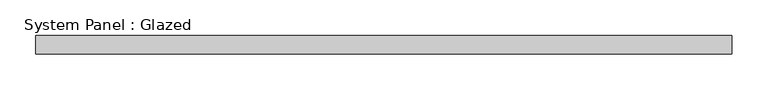
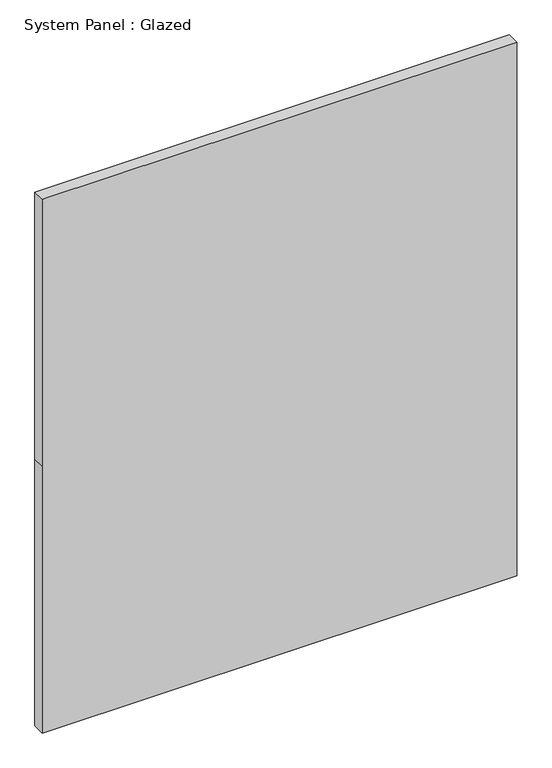
"""IFC4 building model written with IfcOpenShell, lengths in millimetres: plate geometry, System Panel : Glazed."""

import ifcopenshell
import ifcopenshell.guid

model = None  # the IFC model being written
_history = None  # IfcOwnerHistory: only IFC2X3 demands one
_inside = {}  # id of a spatial element -> (the spatial element, [elements in it])
_under = {}  # id of a project, library or spatial element -> (it, [spatial elements below it])
_declared = {}  # id of a project -> (the project, [libraries it declares])
_typed = {}  # id of a type object -> (the type object, [elements of that type])
_made_of = {}  # id of a material, layer set ... -> (it, [elements and type objects made of it])


def new_model(schema):
    """Start an empty IFC model of exactly this schema.

    Asked for "IFC4X3", IfcOpenShell would pick the latest addendum, in which some entities
    have other attributes; the version numbers below select the first issue.
    IFC2X3 requires an IfcOwnerHistory on every rooted entity: one is made here for all.
    """
    global model, _history
    if schema == "IFC4X3":
        model = ifcopenshell.file(schema_version=(4, 3, 0, 0))
    else:
        model = ifcopenshell.file(schema=schema)
    _inside.clear()
    _under.clear()
    _declared.clear()
    _typed.clear()
    _made_of.clear()
    _history = None
    if model.schema == "IFC2X3":
        org = make("IfcOrganization", Name="unknown")
        user = make(
            "IfcPersonAndOrganization",
            ThePerson=make("IfcPerson", FamilyName="unknown"),
            TheOrganization=org,
        )
        app = make(
            "IfcApplication",
            ApplicationDeveloper=org,
            Version="unknown",
            ApplicationFullName="unknown",
            ApplicationIdentifier="unknown",
        )
        _history = make(
            "IfcOwnerHistory",
            OwningUser=user,
            OwningApplication=app,
            ChangeAction="ADDED",
            CreationDate=0,
        )
    return model


def make(cls, **values):
    """One entity of the class cls with the attributes given. An attribute that is None is left unset."""
    return model.create_entity(
        cls, **{name: value for name, value in values.items() if value is not None}
    )


def rooted(cls, **values):
    """An entity with a GlobalId (a new one), such as an element, a storey or a relation."""
    return make(cls, GlobalId=ifcopenshell.guid.new(), OwnerHistory=_history, **values)


def si_unit(unit_type, name, prefix=None):
    """IfcSIUnit, for example si_unit("LENGTHUNIT", "METRE", prefix="MILLI")."""
    return make("IfcSIUnit", UnitType=unit_type, Prefix=prefix, Name=name)


def assignment(units):
    """IfcUnitAssignment: the units of a project."""
    return None if units is None else make("IfcUnitAssignment", Units=units)


def point(xyz):
    """IfcCartesianPoint."""
    return None if xyz is None else make("IfcCartesianPoint", Coordinates=xyz)


def direction(xyz):
    """IfcDirection."""
    return None if xyz is None else make("IfcDirection", DirectionRatios=xyz)


def frame(location, z_axis=None, x_axis=None):
    """IfcAxis2Placement3D, a coordinate frame: its origin and axes. An axis left out is left unset."""
    return make(
        "IfcAxis2Placement3D",
        Location=point(location),
        Axis=direction(z_axis),
        RefDirection=direction(x_axis),
    )


def origin():
    """The frame at (0, 0, 0) with its axes left unset."""
    return frame((0.0, 0.0, 0.0))


def place(relative_to, where):
    """IfcLocalPlacement: puts the frame where relative to a parent placement (None: the world)."""
    return make(
        "IfcLocalPlacement", PlacementRelTo=relative_to, RelativePlacement=where
    )


def context(
    kind, dimensions, precision=None, world=None, true_north=None, identifier=None
):
    """IfcGeometricRepresentationContext, for example the 3D "Model" context."""
    return make(
        "IfcGeometricRepresentationContext",
        ContextIdentifier=identifier,
        ContextType=kind,
        CoordinateSpaceDimension=dimensions,
        Precision=precision,
        WorldCoordinateSystem=world,
        TrueNorth=true_north,
    )


def project(units=None, contexts=None):
    """IfcProject with its units and contexts."""
    return rooted(
        "IfcProject",
        Name="project",
        RepresentationContexts=contexts,
        UnitsInContext=assignment(units),
    )


def spatial(cls, under=None, at=None, **own):
    """A site, building, storey or space (cls), placed at a placement, below another one or the project."""
    s = rooted(cls, ObjectPlacement=at, **own)
    if under is not None:
        _under.setdefault(under.id(), (under, []))[1].append(s)
    return s


def polyline(points):
    """IfcPolyline through the points."""
    return make("IfcPolyline", Points=[point(p) for p in points])


def outline(outer, holes=None, kind="AREA"):
    """IfcArbitraryClosedProfileDef: a profile drawn as a closed curve; with holes, ...WithVoids."""
    if holes is None:
        return make("IfcArbitraryClosedProfileDef", ProfileType=kind, OuterCurve=outer)
    return make(
        "IfcArbitraryProfileDefWithVoids",
        ProfileType=kind,
        OuterCurve=outer,
        InnerCurves=holes,
    )


def extrude(swept, where, along, depth):
    """IfcExtrudedAreaSolid: the profile swept, set in the frame where, extruded along a direction by depth."""
    return make(
        "IfcExtrudedAreaSolid",
        SweptArea=swept,
        Position=where,
        ExtrudedDirection=direction(along),
        Depth=depth,
    )


def shape(context_of_items, identifier, shape_type, items):
    """IfcShapeRepresentation: the items that make up one representation, for example the "Body"."""
    return make(
        "IfcShapeRepresentation",
        ContextOfItems=context_of_items,
        RepresentationIdentifier=identifier,
        RepresentationType=shape_type,
        Items=items,
    )


def source(mapping_origin, context_of_items, identifier, shape_type, items):
    """IfcRepresentationMap: a shape defined once, which mapped items show again and again."""
    return make(
        "IfcRepresentationMap",
        MappingOrigin=mapping_origin,
        MappedRepresentation=shape(context_of_items, identifier, shape_type, items),
    )


def transform(
    local_origin,
    x_axis=None,
    y_axis=None,
    z_axis=None,
    scale=None,
    scale2=None,
    scale3=None,
    uniform=True,
):
    """IfcCartesianTransformationOperator3D, or its non-uniform kind. x_axis, y_axis, z_axis: its Axis1, 2, 3."""
    if uniform:
        return make(
            "IfcCartesianTransformationOperator3D",
            Axis1=direction(x_axis),
            Axis2=direction(y_axis),
            LocalOrigin=point(local_origin),
            Scale=scale,
            Axis3=direction(z_axis),
        )
    return make(
        "IfcCartesianTransformationOperator3DnonUniform",
        Axis1=direction(x_axis),
        Axis2=direction(y_axis),
        LocalOrigin=point(local_origin),
        Scale=scale,
        Axis3=direction(z_axis),
        Scale2=scale2,
        Scale3=scale3,
    )


def mapped(mapping_source, mapping_target):
    """IfcMappedItem: shows the shape of a source again, moved by a transform."""
    return make(
        "IfcMappedItem", MappingSource=mapping_source, MappingTarget=mapping_target
    )


def made_of(thing, what):
    """Note that an element or type object is made of a material, layer set ...; save() writes the relation."""
    if what is not None:
        _made_of.setdefault(what.id(), (what, []))[1].append(thing)
    return thing


def element(
    cls,
    number,
    at=None,
    inside=None,
    cuts=None,
    type_object=None,
    material=None,
    context=None,
    identifier="Body",
    shape_type=None,
    held_by="IfcProductDefinitionShape",
    body=None,
    shapes=None,
    **own,
):
    """One element of the class cls, such as IfcWall. Its Tag is "e" and its number.

    at: its placement. inside: the storey or other place that contains it. cuts: it is an
    opening in that element (IfcRelVoidsElement). A single representation is given by context,
    identifier, shape_type and body (its items); several are given by shapes. held_by: the class
    of the entity that holds the representations. save() writes the other relations.
    """
    e = rooted(cls, Tag="e%d" % number, ObjectPlacement=at, **own)
    if body is not None:
        shapes = [shape(context, identifier, shape_type, body)]
    if shapes is not None:
        e.Representation = make(held_by, Representations=shapes)
    if inside is not None:
        _inside.setdefault(inside.id(), (inside, []))[1].append(e)
    if cuts is not None:
        rooted(
            "IfcRelVoidsElement", RelatingBuildingElement=cuts, RelatedOpeningElement=e
        )
    if type_object is not None:
        _typed.setdefault(type_object.id(), (type_object, []))[1].append(e)
    return made_of(e, material)


def aggregate(whole, parts):
    """IfcRelAggregates: a whole, such as a stair, and the parts it consists of."""
    return rooted("IfcRelAggregates", RelatingObject=whole, RelatedObjects=parts)


def save(model, path):
    """Write the relations noted so far, then the file.

    IfcRelAggregates (storeys below a building ...), IfcRelContainedInSpatialStructure (elements
    in a storey), IfcRelDefinesByType, IfcRelAssociatesMaterial and IfcRelDeclares: one each for
    every whole, place, type object, material and project.
    """
    for whole, parts in _under.values():
        aggregate(whole, parts)
    for where, things in _inside.values():
        rooted(
            "IfcRelContainedInSpatialStructure",
            RelatedElements=things,
            RelatingStructure=where,
        )
    for kind, things in _typed.values():
        rooted("IfcRelDefinesByType", RelatedObjects=things, RelatingType=kind)
    for what, things in _made_of.values():
        rooted("IfcRelAssociatesMaterial", RelatedObjects=things, RelatingMaterial=what)
    for by, libraries in _declared.values():
        rooted("IfcRelDeclares", RelatingContext=by, RelatedDefinitions=libraries)
    model.write(path)


def system_panel_glazed_5449a29c(model_context):
    return source(origin(), model_context, "Body", "SweptSolid", [
        extrude(outline(polyline([(0.0, -485.775), (0.0, 485.775), (577.85, 485.775), (1155.7, 485.775), (1155.7, -485.775), (577.85, -485.775), (0.0, -485.775)])), frame((0.0, -44.45, 0.0), z_axis=(0.0, 1.0, 0.0), x_axis=(0.0, 0.0, 1.0)), (0.0, 0.0, 1.0), 25.4),
    ])


if __name__ == "__main__":
    model = new_model("IFC4")
    model_context = context("Model", 3, world=origin())
    ifc_project = project(units=[si_unit("LENGTHUNIT", "METRE", prefix="MILLI")], contexts=[model_context])
    site = spatial("IfcSite", under=ifc_project)
    building = spatial("IfcBuilding", under=site)
    placement = place(None, origin())
    system_panel_glazed_shape = system_panel_glazed_5449a29c(model_context)
    element("IfcPlate", 1, ObjectType="System Panel : Glazed", at=placement, inside=building, context=model_context, shape_type="MappedRepresentation", body=[
        mapped(system_panel_glazed_shape, transform((0.0, 0.0, 0.0), x_axis=(1.0, 0.0, 0.0), y_axis=(0.0, 1.0, 0.0), z_axis=(0.0, 0.0, 1.0))),
    ])
    save(model, "model.ifc")

# Revit data of these elements
# Project information
#   SR Document GUID = "b4c0fe6c-219c-4d32-b912-4513e366b333"
# Element 1 (IfcPlate, "System Panel : Glazed")
#   Materials on its faces: "Glass"
# Materials
#   "Glass": class "Unassigned", colour RGB 0 0 255, transparency 0.75
